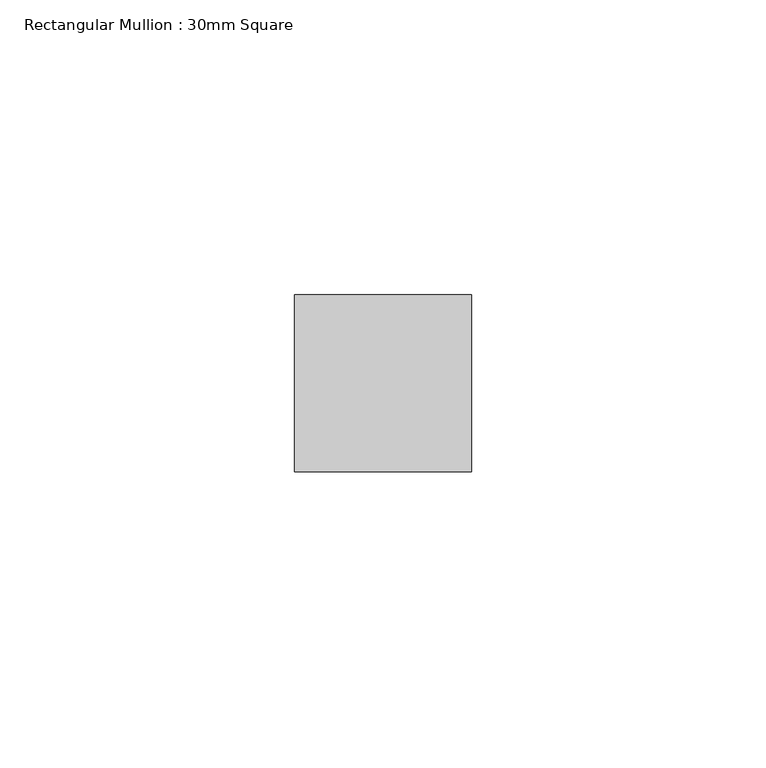
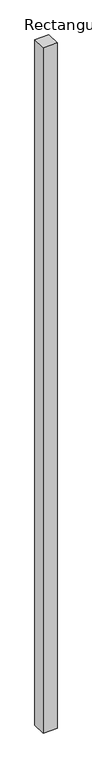
"""IFC4 building model written with IfcOpenShell, lengths in millimetres: member geometry, Rectangular Mullion : 30mm Square."""

from ifc_helpers import new_model, si_unit, frame, origin, place, context, project, spatial, polyline, outline, extrude, source, transform, mapped, element, save


def rectangular_mullion_30mm_square_d4d156d8(model_context):
    return source(origin(), model_context, "Body", "SweptSolid", [
        extrude(outline(polyline([(15.0, 15.0), (15.0, -15.0), (-15.0, -15.0), (-15.0, 15.0), (15.0, 15.0)])), frame((0.0, 0.0, -1549.6931671), z_axis=(0.0, 0.0, 1.0), x_axis=(1.0, 0.0, 0.0)), (0.0, 0.0, 1.0), 1549.6931671),
    ])


if __name__ == "__main__":
    model = new_model("IFC4")
    model_context = context("Model", 3, world=origin())
    ifc_project = project(units=[si_unit("LENGTHUNIT", "METRE", prefix="MILLI")], contexts=[model_context])
    site = spatial("IfcSite", under=ifc_project)
    building = spatial("IfcBuilding", under=site)
    placement = place(None, origin())
    rectangular_mullion_30mm_square_shape = rectangular_mullion_30mm_square_d4d156d8(model_context)
    element("IfcMember", 1, ObjectType="Rectangular Mullion : 30mm Square", at=placement, inside=building, context=model_context, shape_type="MappedRepresentation", body=[
        mapped(rectangular_mullion_30mm_square_shape, transform((0.0, 0.0, 0.0), x_axis=(1.0, 0.0, 0.0), y_axis=(0.0, 1.0, 0.0), z_axis=(0.0, 0.0, 1.0))),
    ])
    save(model, "model.ifc")

# Revit data of these elements
# Type "Rectangular Mullion : 30mm Square"
#   built-in parameter 1007304 = 0.0984252 (stored number, unit not read)
#   built-in parameter 1007301 = 0.0492126 (stored number, unit not read)
#   built-in parameter 1007300 = 0.0492126 (stored number, unit not read)
# Element 1 (IfcMember, "Rectangular Mullion : 30mm Square")
#   Materials on its faces: "Aluminum"
# Materials
#   "Aluminum": class "Metal", colour RGB 244 244 244, transparency 0, Description = "Aluminum 6061", Cost = 0
